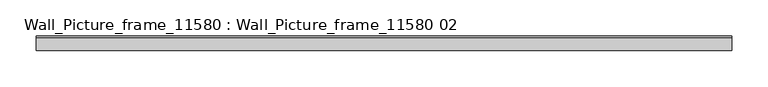
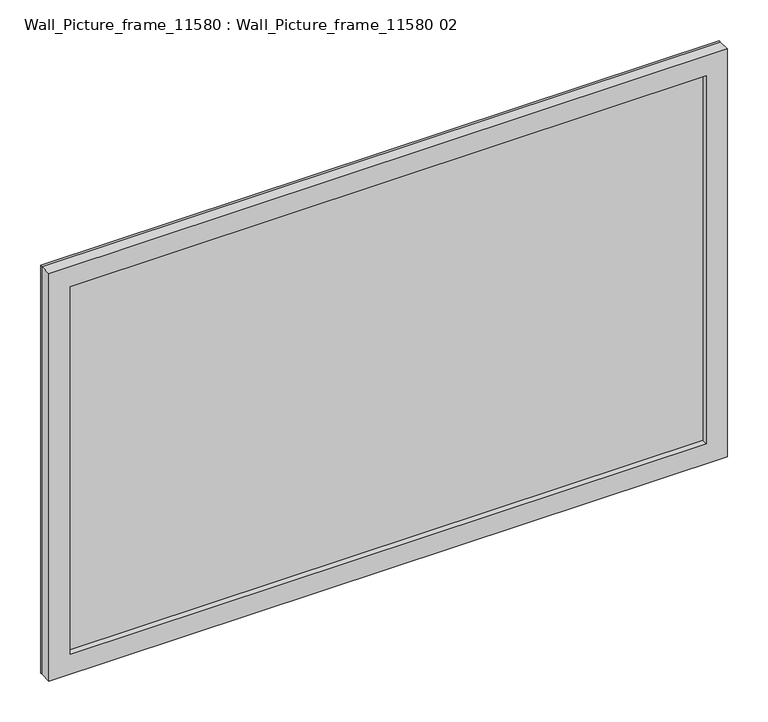
"""IFC4 building model written with IfcOpenShell, lengths in millimetres: furniture geometry, Wall_Picture_frame_11580 : Wall_Picture_frame_11580 02."""

import ifcopenshell
import ifcopenshell.guid

model = None  # the IFC model being written
_history = None  # IfcOwnerHistory: only IFC2X3 demands one
_inside = {}  # id of a spatial element -> (the spatial element, [elements in it])
_under = {}  # id of a project, library or spatial element -> (it, [spatial elements below it])
_declared = {}  # id of a project -> (the project, [libraries it declares])
_typed = {}  # id of a type object -> (the type object, [elements of that type])
_made_of = {}  # id of a material, layer set ... -> (it, [elements and type objects made of it])


def new_model(schema):
    """Start an empty IFC model of exactly this schema.

    Asked for "IFC4X3", IfcOpenShell would pick the latest addendum, in which some entities
    have other attributes; the version numbers below select the first issue.
    IFC2X3 requires an IfcOwnerHistory on every rooted entity: one is made here for all.
    """
    global model, _history
    if schema == "IFC4X3":
        model = ifcopenshell.file(schema_version=(4, 3, 0, 0))
    else:
        model = ifcopenshell.file(schema=schema)
    _inside.clear()
    _under.clear()
    _declared.clear()
    _typed.clear()
    _made_of.clear()
    _history = None
    if model.schema == "IFC2X3":
        org = make("IfcOrganization", Name="unknown")
        user = make(
            "IfcPersonAndOrganization",
            ThePerson=make("IfcPerson", FamilyName="unknown"),
            TheOrganization=org,
        )
        app = make(
            "IfcApplication",
            ApplicationDeveloper=org,
            Version="unknown",
            ApplicationFullName="unknown",
            ApplicationIdentifier="unknown",
        )
        _history = make(
            "IfcOwnerHistory",
            OwningUser=user,
            OwningApplication=app,
            ChangeAction="ADDED",
            CreationDate=0,
        )
    return model


def make(cls, **values):
    """One entity of the class cls with the attributes given. An attribute that is None is left unset."""
    return model.create_entity(
        cls, **{name: value for name, value in values.items() if value is not None}
    )


def rooted(cls, **values):
    """An entity with a GlobalId (a new one), such as an element, a storey or a relation."""
    return make(cls, GlobalId=ifcopenshell.guid.new(), OwnerHistory=_history, **values)


def si_unit(unit_type, name, prefix=None):
    """IfcSIUnit, for example si_unit("LENGTHUNIT", "METRE", prefix="MILLI")."""
    return make("IfcSIUnit", UnitType=unit_type, Prefix=prefix, Name=name)


def assignment(units):
    """IfcUnitAssignment: the units of a project."""
    return None if units is None else make("IfcUnitAssignment", Units=units)


def point(xyz):
    """IfcCartesianPoint."""
    return None if xyz is None else make("IfcCartesianPoint", Coordinates=xyz)


def direction(xyz):
    """IfcDirection."""
    return None if xyz is None else make("IfcDirection", DirectionRatios=xyz)


def frame(location, z_axis=None, x_axis=None):
    """IfcAxis2Placement3D, a coordinate frame: its origin and axes. An axis left out is left unset."""
    return make(
        "IfcAxis2Placement3D",
        Location=point(location),
        Axis=direction(z_axis),
        RefDirection=direction(x_axis),
    )


def origin():
    """The frame at (0, 0, 0) with its axes left unset."""
    return frame((0.0, 0.0, 0.0))


def origin_with_axes():
    """The frame at (0, 0, 0) with the z axis (0, 0, 1) and the x axis (1, 0, 0) written out."""
    return frame((0.0, 0.0, 0.0), z_axis=(0.0, 0.0, 1.0), x_axis=(1.0, 0.0, 0.0))


def place(relative_to, where):
    """IfcLocalPlacement: puts the frame where relative to a parent placement (None: the world)."""
    return make(
        "IfcLocalPlacement", PlacementRelTo=relative_to, RelativePlacement=where
    )


def context(
    kind, dimensions, precision=None, world=None, true_north=None, identifier=None
):
    """IfcGeometricRepresentationContext, for example the 3D "Model" context."""
    return make(
        "IfcGeometricRepresentationContext",
        ContextIdentifier=identifier,
        ContextType=kind,
        CoordinateSpaceDimension=dimensions,
        Precision=precision,
        WorldCoordinateSystem=world,
        TrueNorth=true_north,
    )


def project(units=None, contexts=None):
    """IfcProject with its units and contexts."""
    return rooted(
        "IfcProject",
        Name="project",
        RepresentationContexts=contexts,
        UnitsInContext=assignment(units),
    )


def spatial(cls, under=None, at=None, **own):
    """A site, building, storey or space (cls), placed at a placement, below another one or the project."""
    s = rooted(cls, ObjectPlacement=at, **own)
    if under is not None:
        _under.setdefault(under.id(), (under, []))[1].append(s)
    return s


def polyline(points):
    """IfcPolyline through the points."""
    return make("IfcPolyline", Points=[point(p) for p in points])


def outline(outer, holes=None, kind="AREA"):
    """IfcArbitraryClosedProfileDef: a profile drawn as a closed curve; with holes, ...WithVoids."""
    if holes is None:
        return make("IfcArbitraryClosedProfileDef", ProfileType=kind, OuterCurve=outer)
    return make(
        "IfcArbitraryProfileDefWithVoids",
        ProfileType=kind,
        OuterCurve=outer,
        InnerCurves=holes,
    )


def extrude(swept, where, along, depth):
    """IfcExtrudedAreaSolid: the profile swept, set in the frame where, extruded along a direction by depth."""
    return make(
        "IfcExtrudedAreaSolid",
        SweptArea=swept,
        Position=where,
        ExtrudedDirection=direction(along),
        Depth=depth,
    )


def shape(context_of_items, identifier, shape_type, items):
    """IfcShapeRepresentation: the items that make up one representation, for example the "Body"."""
    return make(
        "IfcShapeRepresentation",
        ContextOfItems=context_of_items,
        RepresentationIdentifier=identifier,
        RepresentationType=shape_type,
        Items=items,
    )


def source(mapping_origin, context_of_items, identifier, shape_type, items):
    """IfcRepresentationMap: a shape defined once, which mapped items show again and again."""
    return make(
        "IfcRepresentationMap",
        MappingOrigin=mapping_origin,
        MappedRepresentation=shape(context_of_items, identifier, shape_type, items),
    )


def transform(
    local_origin,
    x_axis=None,
    y_axis=None,
    z_axis=None,
    scale=None,
    scale2=None,
    scale3=None,
    uniform=True,
):
    """IfcCartesianTransformationOperator3D, or its non-uniform kind. x_axis, y_axis, z_axis: its Axis1, 2, 3."""
    if uniform:
        return make(
            "IfcCartesianTransformationOperator3D",
            Axis1=direction(x_axis),
            Axis2=direction(y_axis),
            LocalOrigin=point(local_origin),
            Scale=scale,
            Axis3=direction(z_axis),
        )
    return make(
        "IfcCartesianTransformationOperator3DnonUniform",
        Axis1=direction(x_axis),
        Axis2=direction(y_axis),
        LocalOrigin=point(local_origin),
        Scale=scale,
        Axis3=direction(z_axis),
        Scale2=scale2,
        Scale3=scale3,
    )


def mapped(mapping_source, mapping_target):
    """IfcMappedItem: shows the shape of a source again, moved by a transform."""
    return make(
        "IfcMappedItem", MappingSource=mapping_source, MappingTarget=mapping_target
    )


def made_of(thing, what):
    """Note that an element or type object is made of a material, layer set ...; save() writes the relation."""
    if what is not None:
        _made_of.setdefault(what.id(), (what, []))[1].append(thing)
    return thing


def element(
    cls,
    number,
    at=None,
    inside=None,
    cuts=None,
    type_object=None,
    material=None,
    context=None,
    identifier="Body",
    shape_type=None,
    held_by="IfcProductDefinitionShape",
    body=None,
    shapes=None,
    **own,
):
    """One element of the class cls, such as IfcWall. Its Tag is "e" and its number.

    at: its placement. inside: the storey or other place that contains it. cuts: it is an
    opening in that element (IfcRelVoidsElement). A single representation is given by context,
    identifier, shape_type and body (its items); several are given by shapes. held_by: the class
    of the entity that holds the representations. save() writes the other relations.
    """
    e = rooted(cls, Tag="e%d" % number, ObjectPlacement=at, **own)
    if body is not None:
        shapes = [shape(context, identifier, shape_type, body)]
    if shapes is not None:
        e.Representation = make(held_by, Representations=shapes)
    if inside is not None:
        _inside.setdefault(inside.id(), (inside, []))[1].append(e)
    if cuts is not None:
        rooted(
            "IfcRelVoidsElement", RelatingBuildingElement=cuts, RelatedOpeningElement=e
        )
    if type_object is not None:
        _typed.setdefault(type_object.id(), (type_object, []))[1].append(e)
    return made_of(e, material)


def aggregate(whole, parts):
    """IfcRelAggregates: a whole, such as a stair, and the parts it consists of."""
    return rooted("IfcRelAggregates", RelatingObject=whole, RelatedObjects=parts)


def save(model, path):
    """Write the relations noted so far, then the file.

    IfcRelAggregates (storeys below a building ...), IfcRelContainedInSpatialStructure (elements
    in a storey), IfcRelDefinesByType, IfcRelAssociatesMaterial and IfcRelDeclares: one each for
    every whole, place, type object, material and project.
    """
    for whole, parts in _under.values():
        aggregate(whole, parts)
    for where, things in _inside.values():
        rooted(
            "IfcRelContainedInSpatialStructure",
            RelatedElements=things,
            RelatingStructure=where,
        )
    for kind, things in _typed.values():
        rooted("IfcRelDefinesByType", RelatedObjects=things, RelatingType=kind)
    for what, things in _made_of.values():
        rooted("IfcRelAssociatesMaterial", RelatedObjects=things, RelatingMaterial=what)
    for by, libraries in _declared.values():
        rooted("IfcRelDeclares", RelatingContext=by, RelatedDefinitions=libraries)
    model.write(path)


def wall_picture_frame_11580_wall_picture_frame_11580_02_aef4a011(model_context):
    return source(origin(), model_context, "Body", "SweptSolid", [
        extrude(outline(polyline([(930.0, -12.0), (30.0, -12.0), (30.0, -10.0), (930.0, -10.0), (930.0, -12.0)])), frame((0.0, 0.0, 30.0), z_axis=(0.0, 0.0, 1.0), x_axis=(1.0, 0.0, 0.0)), (0.0, 0.0, 1.0), 550.0),
        extrude(outline(polyline([(855.0, -5.0), (105.0, -5.0), (105.0, -3.0), (855.0, -3.0), (855.0, -5.0)])), frame((0.0, 0.0, 105.0), z_axis=(0.0, 0.0, 1.0), x_axis=(1.0, 0.0, 0.0)), (0.0, 0.0, 1.0), 400.0),
        extrude(outline(polyline([(580.0, 930.0), (580.0, 30.0), (30.0, 30.0), (30.0, 930.0), (580.0, 930.0)]), holes=[polyline([(505.0, 855.0), (105.0, 855.0), (105.0, 105.0), (505.0, 105.0), (505.0, 855.0)])]), frame((0.0, -9.0, 0.0), z_axis=(0.0, 1.0, 0.0), x_axis=(0.0, 0.0, 1.0)), (0.0, 0.0, 1.0), 6.0),
        extrude(outline(polyline([(610.0, 0.0), (0.0, 0.0), (0.0, 960.0), (610.0, 960.0), (610.0, 0.0)]), holes=[polyline([(580.0, 930.0), (30.0, 930.0), (30.0, 30.0), (580.0, 30.0), (580.0, 930.0)])]), frame((0.0, -20.0, 0.0), z_axis=(0.0, 1.0, 0.0), x_axis=(0.0, 0.0, 1.0)), (0.0, 0.0, 1.0), 17.0),
        extrude(outline(polyline([(960.0, -3.0), (0.0, -3.0), (0.0, 0.0), (960.0, 0.0), (960.0, -3.0)])), origin_with_axes(), (0.0, 0.0, 1.0), 610.0),
    ])


if __name__ == "__main__":
    model = new_model("IFC4")
    model_context = context("Model", 3, world=origin())
    ifc_project = project(units=[si_unit("LENGTHUNIT", "METRE", prefix="MILLI")], contexts=[model_context])
    site = spatial("IfcSite", under=ifc_project)
    building = spatial("IfcBuilding", under=site)
    placement = place(None, origin())
    wall_picture_frame_11580_wall_picture_frame_11580_02_shape = wall_picture_frame_11580_wall_picture_frame_11580_02_aef4a011(model_context)
    element("IfcFurniture", 1, ObjectType="Wall_Picture_frame_11580 : Wall_Picture_frame_11580 02", at=placement, inside=building, context=model_context, shape_type="MappedRepresentation", body=[
        mapped(wall_picture_frame_11580_wall_picture_frame_11580_02_shape, transform((0.0, 0.0, 0.0), x_axis=(1.0, 0.0, 0.0), y_axis=(0.0, 1.0, 0.0), z_axis=(0.0, 0.0, 1.0))),
    ])
    save(model, "model.ifc")

# Revit data of these elements
# Type "Wall_Picture_frame_11580 : Wall_Picture_frame_11580 02"
#   Width [instance default] = 960 mm
#   Picture width [instance default] = 750 mm
#   Picture height [instance default] = 400 mm
#   Passepartout width [instance default] = 75 mm
#   Height [instance default] = 610 mm
#   Frame width [instance default] = 30 mm
#   Picture [instance default] = none
#   Passe-partout = Picture-Passepartout
#   Front glass = Picture-front glass
#   Frame = Picture-frame
#   Default Elevation = 0
# Element 1 (IfcFurniture, "Wall_Picture_frame_11580 : Wall_Picture_frame_11580 02")
#   Materials on its faces: "Picture-frame", "Picture-Passepartout", "Picture-front glass"
# Materials
#   "Picture-Passepartout": class "Miscellaneous", colour RGB 127 127 127, transparency 0
#   "Picture-front glass": class "Glass", colour RGB 250 250 250, transparency 0.9
#   "Picture-frame": class "Miscellaneous", colour RGB 3 3 3, transparency 0
